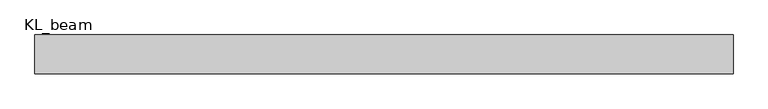
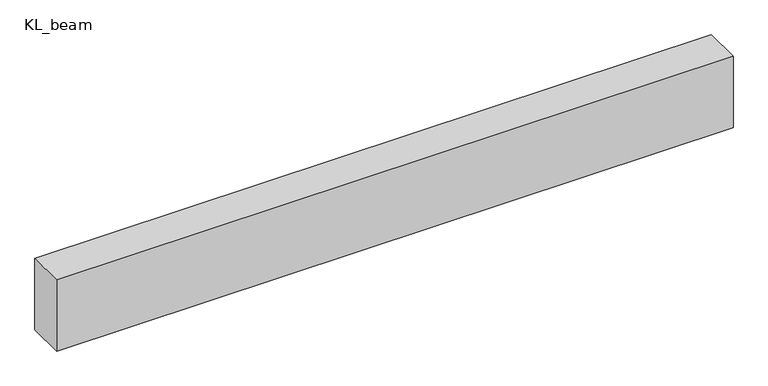
"""IFC4 building model written with IfcOpenShell, lengths in millimetres: beam geometry, 混凝土 - 矩形梁 : KL_beam."""

from ifc_helpers import new_model, si_unit, frame, origin, place, context, project, spatial, polyline, outline, extrude, source, transform, mapped, element, save


def kl_beam_3ef5503e(model_context):
    return source(origin(), model_context, "Body", "SweptSolid", [
        extrude(outline(polyline([(3600.0, 200.0), (3600.0, -200.0), (-3600.0, -200.0), (-3600.0, 200.0), (3600.0, 200.0)])), frame((0.0, 0.0, -400.0), z_axis=(0.0, 0.0, 1.0), x_axis=(1.0, 0.0, 0.0)), (0.0, 0.0, 1.0), 800.0),
    ])


if __name__ == "__main__":
    model = new_model("IFC4")
    model_context = context("Model", 3, world=origin())
    ifc_project = project(units=[si_unit("LENGTHUNIT", "METRE", prefix="MILLI")], contexts=[model_context])
    site = spatial("IfcSite", under=ifc_project)
    building = spatial("IfcBuilding", under=site)
    placement = place(None, origin())
    kl_beam_shape = kl_beam_3ef5503e(model_context)
    element("IfcBeam", 1, ObjectType="混凝土 - 矩形梁 : KL_beam", at=placement, inside=building, context=model_context, shape_type="MappedRepresentation", body=[
        mapped(kl_beam_shape, transform((0.0, 0.0, 0.0), x_axis=(1.0, 0.0, 0.0), y_axis=(0.0, 1.0, 0.0), z_axis=(0.0, 0.0, 1.0))),
    ])
    save(model, "model.ifc")

# Revit data of these elements
# Type "混凝土 - 矩形梁 : KL_beam"
#   Length [instance default] = 1524 mm
#   b = 400 mm
#   h = 800 mm
#   Structural Material [instance default] = 混凝土 - 现场浇注混凝土
#   Assembly Code = ""
# Element 1 (IfcBeam, "混凝土 - 矩形梁 : KL_beam")
#   Structural Material = none
# Materials
#   "混凝土 - 现场浇注混凝土": class "混凝土", colour RGB 192 192 192, transparency 0
